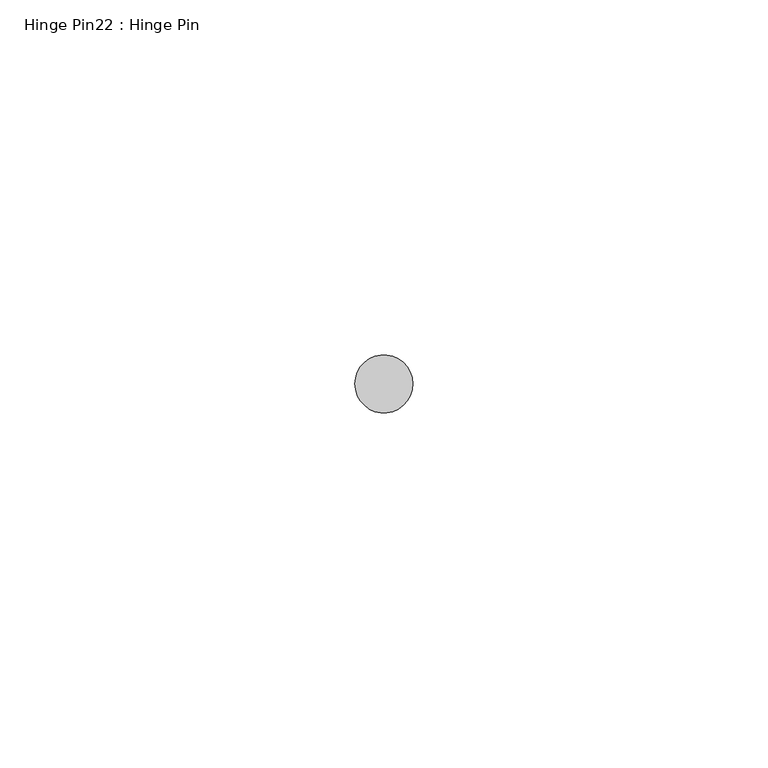
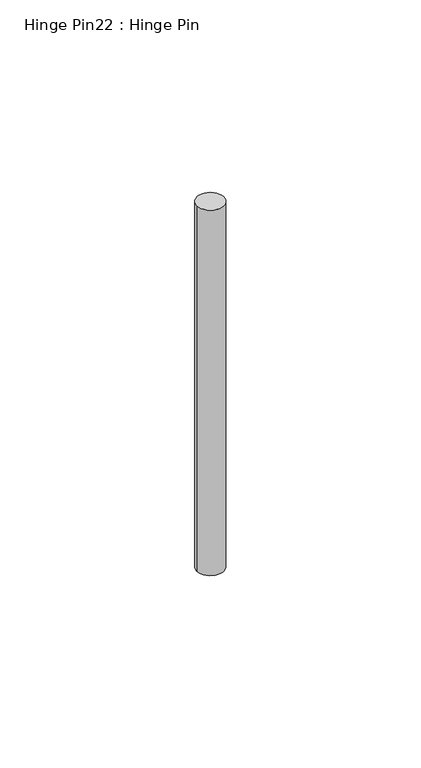
"""IFC4 building model written with IfcOpenShell, lengths in millimetres: proxy geometry, Hinge Pin22 : Hinge Pin."""

from ifc_helpers import new_model, si_unit, point, frame, frame_2d, origin, place, context, project, spatial, circle_curve, trimmed, segment, composite_curve, outline, extrude, source, transform, mapped, element, save


def hinge_pin22_hinge_pin_b100999e(model_context):
    return source(origin(), model_context, "Body", "SweptSolid", [
        extrude(outline(composite_curve([segment(trimmed(circle_curve(frame_2d((587319.1320739, -536310.3652841)), 4.0894), [point((587315.0426739, -536310.3652841))], [point((587323.2214739, -536310.3652841))], False, "CARTESIAN"), True, "CONTINUOUS"), segment(trimmed(circle_curve(frame_2d((587319.1320739, -536310.3652841)), 4.0894), [point((587323.2214739, -536310.3652841))], [point((587315.0426739, -536310.3652841))], False, "CARTESIAN"), True, "CONTINUOUS")], self_intersect=False)), frame((0.0, 0.0, 1941.3140625), z_axis=(0.0, 0.0, 1.0), x_axis=(1.0, 0.0, 0.0)), (0.0, 0.0, 1.0), 117.871875),
    ])


if __name__ == "__main__":
    model = new_model("IFC4")
    model_context = context("Model", 3, world=origin())
    ifc_project = project(units=[si_unit("LENGTHUNIT", "METRE", prefix="MILLI")], contexts=[model_context])
    site = spatial("IfcSite", under=ifc_project)
    building = spatial("IfcBuilding", under=site)
    placement = place(None, origin())
    hinge_pin22_hinge_pin_shape = hinge_pin22_hinge_pin_b100999e(model_context)
    element("IfcBuildingElementProxy", 1, Name="Hinge Pin22 : Hinge Pin", ObjectType="Hinge Pin22 : Hinge Pin", at=placement, inside=building, context=model_context, shape_type="MappedRepresentation", body=[
        mapped(hinge_pin22_hinge_pin_shape, transform((0.0, 0.0, 0.0), x_axis=(1.0, 0.0, 0.0), y_axis=(0.0, 1.0, 0.0), z_axis=(0.0, 0.0, 1.0))),
    ])
    save(model, "model.ifc")

# Revit data of these elements
# Element 1 (IfcBuildingElementProxy, "Hinge Pin22 : Hinge Pin")
#   Materials on its faces: "6\"X6\" WELD-ON STL BUTT HINGE"
# Materials
#   "6\"X6\" WELD-ON STL BUTT HINGE": class "Metal", colour RGB 189 187 185, transparency 0, Description = "Carbon steel", Cost = 0
